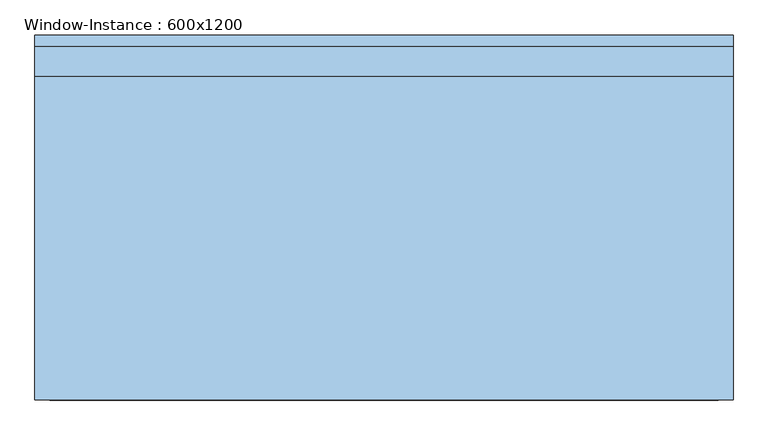
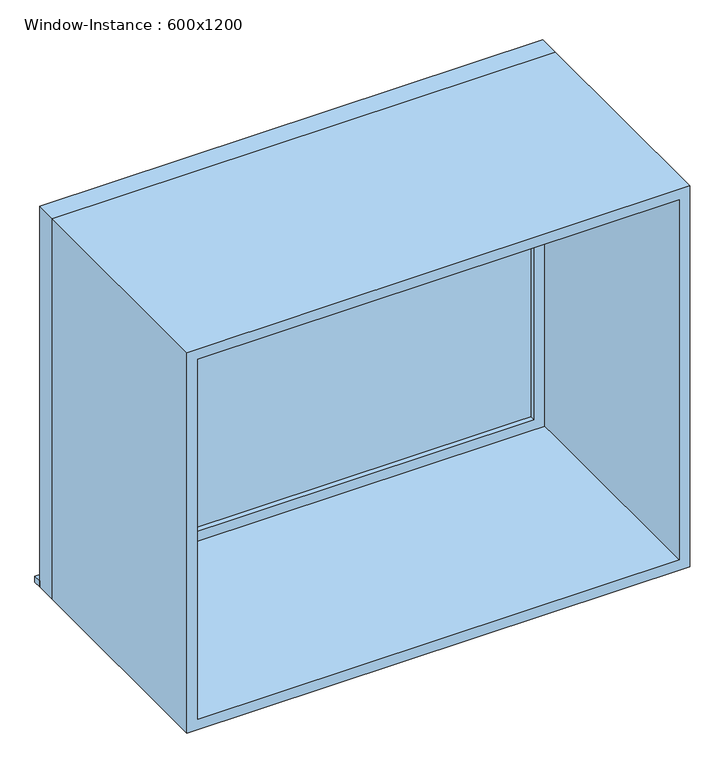
"""IFC4 building model written with IfcOpenShell, lengths in millimetres: window geometry, Window-Instance : 600x1200."""

from ifc_helpers import new_model, si_unit, frame, origin, place, context, project, spatial, polyline, outline, extrude, source, transform, mapped, element, save


def window_instance_600x1200_e6ff42af(model_context):
    return source(origin(), model_context, "Body", "SweptSolid", [
        extrude(outline(polyline([(-788.1, 405.4), (711.9, 405.4), (711.9, 380.0), (-788.1, 380.0), (-788.1, 405.4)])), frame((0.0, 0.0, 900.0), z_axis=(0.0, 0.0, 1.0), x_axis=(1.0, 0.0, 0.0)), (0.0, 0.0, 1.0), 19.05),
        extrude(outline(polyline([(648.4, 331.425), (-724.6, 331.425), (-724.6, 344.125), (648.4, 344.125), (648.4, 331.425)])), frame((0.0, 0.0, 963.5), z_axis=(0.0, 0.0, 1.0), x_axis=(1.0, 0.0, 0.0)), (0.0, 0.0, 1.0), 1073.0),
        extrude(outline(polyline([(2080.95, -769.05), (919.05, -769.05), (919.05, 692.85), (2080.95, 692.85), (2080.95, -769.05)]), holes=[polyline([(2036.5, -724.6), (2036.5, 648.4), (963.5, 648.4), (963.5, -724.6), (2036.5, -724.6)])]), frame((0.0, 315.55, 0.0), z_axis=(0.0, 1.0, 0.0), x_axis=(0.0, 0.0, 1.0)), (0.0, 0.0, 1.0), 44.45),
        extrude(outline(polyline([(2100.0, -788.1), (900.0, -788.1), (900.0, 711.9), (2100.0, 711.9), (2100.0, -788.1)]), holes=[polyline([(2068.25, -756.35), (2068.25, 680.15), (931.75, 680.15), (931.75, -756.35), (2068.25, -756.35)])]), frame((0.0, -380.0, 0.0), z_axis=(0.0, 1.0, 0.0), x_axis=(0.0, 0.0, 1.0)), (0.0, 0.0, 1.0), 695.55),
        extrude(outline(polyline([(2100.0, 711.9), (2100.0, -788.1), (900.0, -788.1), (900.0, 711.9), (2100.0, 711.9)]), holes=[polyline([(2080.95, 692.85), (919.05, 692.85), (919.05, -769.05), (2080.95, -769.05), (2080.95, 692.85)])]), frame((0.0, 315.55, 0.0), z_axis=(0.0, 1.0, 0.0), x_axis=(0.0, 0.0, 1.0)), (0.0, 0.0, 1.0), 64.45),
    ])


if __name__ == "__main__":
    model = new_model("IFC4")
    model_context = context("Model", 3, world=origin())
    ifc_project = project(units=[si_unit("LENGTHUNIT", "METRE", prefix="MILLI")], contexts=[model_context])
    site = spatial("IfcSite", under=ifc_project)
    building = spatial("IfcBuilding", under=site)
    placement = place(None, origin())
    window_instance_600x1200_shape = window_instance_600x1200_e6ff42af(model_context)
    element("IfcWindow", 1, ObjectType="Window-Instance : 600x1200", at=placement, inside=building, context=model_context, shape_type="MappedRepresentation", body=[
        mapped(window_instance_600x1200_shape, transform((0.0, 0.0, 0.0), x_axis=(1.0, 0.0, 0.0), y_axis=(0.0, 1.0, 0.0), z_axis=(0.0, 0.0, 1.0))),
    ])
    save(model, "model.ifc")

# Revit data of these elements
# Type "Window-Instance : 600x1200"
#   Type Mark = "7"
#   Construction Type Id = "GSP4R"
#   Assembly Code = "B2020100"
#   Analytic Construction = "1/8 in Pilkington single glazing"
#   Visual Light Transmittance = 0.9
#   Thermal Resistance (R) = 0.149095 (m²·K)/W
#   Solar Heat Gain Coefficient = 0.86
#   Heat Transfer Coefficient (U) = 6.70716 W/(m²·K)
#   Height [instance default] = 1200 mm
#   Default Sill Height = 900 mm
#   Width [instance default] = 600 mm
#   Window Inset = 20 mm
#   Glass Pane Material = WW-EC-GL-Storefront
#   Sash Material = WW-EC-RGB-White
#   Wall Closure = (empty or 0)
# Element 1 (IfcWindow, "Window-Instance : 600x1200")
#   Width = 1500 mm
#   Materials on its faces: "WW-EC-RGB-White", "WW-EC-GL-Storefront"
# Materials
#   "WW-EC-GL-Storefront": class "Glass", colour RGB 236 240 239, transparency 0.85, Description = "Storefront Glass", Cost = 0
#   "WW-EC-RGB-White": class "Generic", colour RGB 255 255 255, transparency 0, Comments = "If region requests off-white, swith asset color to RGB 231-228-220", Description = "Generic Color", Cost = 0
